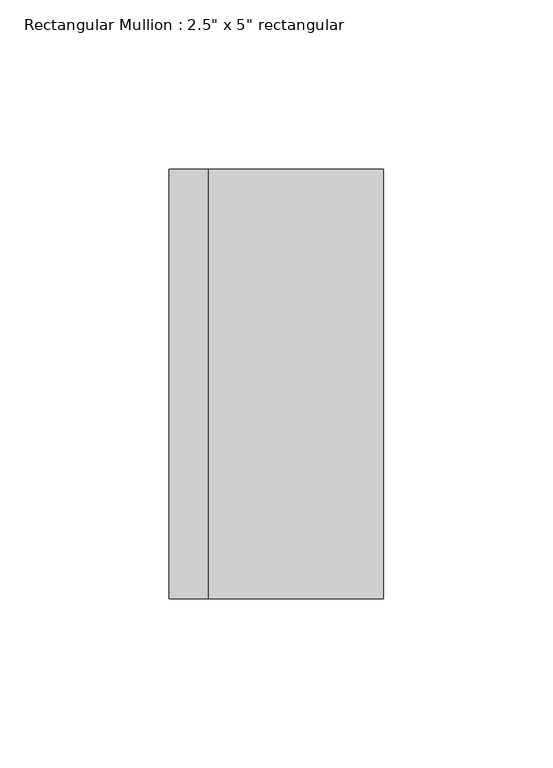
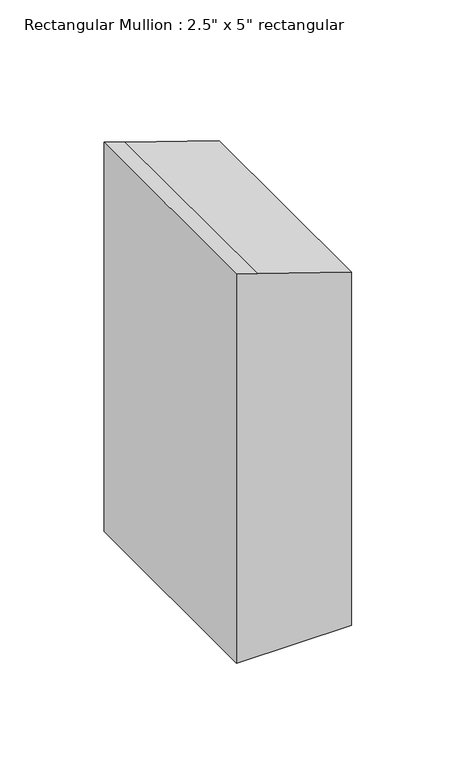
"""IFC4 building model written with IfcOpenShell, lengths in millimetres: member geometry."""

import ifcopenshell
import ifcopenshell.guid

model = None  # the IFC model being written
_history = None  # IfcOwnerHistory: only IFC2X3 demands one
_inside = {}  # id of a spatial element -> (the spatial element, [elements in it])
_under = {}  # id of a project, library or spatial element -> (it, [spatial elements below it])
_declared = {}  # id of a project -> (the project, [libraries it declares])
_typed = {}  # id of a type object -> (the type object, [elements of that type])
_made_of = {}  # id of a material, layer set ... -> (it, [elements and type objects made of it])


def new_model(schema):
    """Start an empty IFC model of exactly this schema.

    Asked for "IFC4X3", IfcOpenShell would pick the latest addendum, in which some entities
    have other attributes; the version numbers below select the first issue.
    IFC2X3 requires an IfcOwnerHistory on every rooted entity: one is made here for all.
    """
    global model, _history
    if schema == "IFC4X3":
        model = ifcopenshell.file(schema_version=(4, 3, 0, 0))
    else:
        model = ifcopenshell.file(schema=schema)
    _inside.clear()
    _under.clear()
    _declared.clear()
    _typed.clear()
    _made_of.clear()
    _history = None
    if model.schema == "IFC2X3":
        org = make("IfcOrganization", Name="unknown")
        user = make(
            "IfcPersonAndOrganization",
            ThePerson=make("IfcPerson", FamilyName="unknown"),
            TheOrganization=org,
        )
        app = make(
            "IfcApplication",
            ApplicationDeveloper=org,
            Version="unknown",
            ApplicationFullName="unknown",
            ApplicationIdentifier="unknown",
        )
        _history = make(
            "IfcOwnerHistory",
            OwningUser=user,
            OwningApplication=app,
            ChangeAction="ADDED",
            CreationDate=0,
        )
    return model


def make(cls, **values):
    """One entity of the class cls with the attributes given. An attribute that is None is left unset."""
    return model.create_entity(
        cls, **{name: value for name, value in values.items() if value is not None}
    )


def rooted(cls, **values):
    """An entity with a GlobalId (a new one), such as an element, a storey or a relation."""
    return make(cls, GlobalId=ifcopenshell.guid.new(), OwnerHistory=_history, **values)


def si_unit(unit_type, name, prefix=None):
    """IfcSIUnit, for example si_unit("LENGTHUNIT", "METRE", prefix="MILLI")."""
    return make("IfcSIUnit", UnitType=unit_type, Prefix=prefix, Name=name)


def assignment(units):
    """IfcUnitAssignment: the units of a project."""
    return None if units is None else make("IfcUnitAssignment", Units=units)


def point(xyz):
    """IfcCartesianPoint."""
    return None if xyz is None else make("IfcCartesianPoint", Coordinates=xyz)


def direction(xyz):
    """IfcDirection."""
    return None if xyz is None else make("IfcDirection", DirectionRatios=xyz)


def frame(location, z_axis=None, x_axis=None):
    """IfcAxis2Placement3D, a coordinate frame: its origin and axes. An axis left out is left unset."""
    return make(
        "IfcAxis2Placement3D",
        Location=point(location),
        Axis=direction(z_axis),
        RefDirection=direction(x_axis),
    )


def origin():
    """The frame at (0, 0, 0) with its axes left unset."""
    return frame((0.0, 0.0, 0.0))


def place(relative_to, where):
    """IfcLocalPlacement: puts the frame where relative to a parent placement (None: the world)."""
    return make(
        "IfcLocalPlacement", PlacementRelTo=relative_to, RelativePlacement=where
    )


def context(
    kind, dimensions, precision=None, world=None, true_north=None, identifier=None
):
    """IfcGeometricRepresentationContext, for example the 3D "Model" context."""
    return make(
        "IfcGeometricRepresentationContext",
        ContextIdentifier=identifier,
        ContextType=kind,
        CoordinateSpaceDimension=dimensions,
        Precision=precision,
        WorldCoordinateSystem=world,
        TrueNorth=true_north,
    )


def project(units=None, contexts=None):
    """IfcProject with its units and contexts."""
    return rooted(
        "IfcProject",
        Name="project",
        RepresentationContexts=contexts,
        UnitsInContext=assignment(units),
    )


def spatial(cls, under=None, at=None, **own):
    """A site, building, storey or space (cls), placed at a placement, below another one or the project."""
    s = rooted(cls, ObjectPlacement=at, **own)
    if under is not None:
        _under.setdefault(under.id(), (under, []))[1].append(s)
    return s


def polyline(points):
    """IfcPolyline through the points."""
    return make("IfcPolyline", Points=[point(p) for p in points])


def outline(outer, holes=None, kind="AREA"):
    """IfcArbitraryClosedProfileDef: a profile drawn as a closed curve; with holes, ...WithVoids."""
    if holes is None:
        return make("IfcArbitraryClosedProfileDef", ProfileType=kind, OuterCurve=outer)
    return make(
        "IfcArbitraryProfileDefWithVoids",
        ProfileType=kind,
        OuterCurve=outer,
        InnerCurves=holes,
    )


def extrude(swept, where, along, depth):
    """IfcExtrudedAreaSolid: the profile swept, set in the frame where, extruded along a direction by depth."""
    return make(
        "IfcExtrudedAreaSolid",
        SweptArea=swept,
        Position=where,
        ExtrudedDirection=direction(along),
        Depth=depth,
    )


def shape(context_of_items, identifier, shape_type, items):
    """IfcShapeRepresentation: the items that make up one representation, for example the "Body"."""
    return make(
        "IfcShapeRepresentation",
        ContextOfItems=context_of_items,
        RepresentationIdentifier=identifier,
        RepresentationType=shape_type,
        Items=items,
    )


def source(mapping_origin, context_of_items, identifier, shape_type, items):
    """IfcRepresentationMap: a shape defined once, which mapped items show again and again."""
    return make(
        "IfcRepresentationMap",
        MappingOrigin=mapping_origin,
        MappedRepresentation=shape(context_of_items, identifier, shape_type, items),
    )


def transform(
    local_origin,
    x_axis=None,
    y_axis=None,
    z_axis=None,
    scale=None,
    scale2=None,
    scale3=None,
    uniform=True,
):
    """IfcCartesianTransformationOperator3D, or its non-uniform kind. x_axis, y_axis, z_axis: its Axis1, 2, 3."""
    if uniform:
        return make(
            "IfcCartesianTransformationOperator3D",
            Axis1=direction(x_axis),
            Axis2=direction(y_axis),
            LocalOrigin=point(local_origin),
            Scale=scale,
            Axis3=direction(z_axis),
        )
    return make(
        "IfcCartesianTransformationOperator3DnonUniform",
        Axis1=direction(x_axis),
        Axis2=direction(y_axis),
        LocalOrigin=point(local_origin),
        Scale=scale,
        Axis3=direction(z_axis),
        Scale2=scale2,
        Scale3=scale3,
    )


def mapped(mapping_source, mapping_target):
    """IfcMappedItem: shows the shape of a source again, moved by a transform."""
    return make(
        "IfcMappedItem", MappingSource=mapping_source, MappingTarget=mapping_target
    )


def made_of(thing, what):
    """Note that an element or type object is made of a material, layer set ...; save() writes the relation."""
    if what is not None:
        _made_of.setdefault(what.id(), (what, []))[1].append(thing)
    return thing


def element(
    cls,
    number,
    at=None,
    inside=None,
    cuts=None,
    type_object=None,
    material=None,
    context=None,
    identifier="Body",
    shape_type=None,
    held_by="IfcProductDefinitionShape",
    body=None,
    shapes=None,
    **own,
):
    """One element of the class cls, such as IfcWall. Its Tag is "e" and its number.

    at: its placement. inside: the storey or other place that contains it. cuts: it is an
    opening in that element (IfcRelVoidsElement). A single representation is given by context,
    identifier, shape_type and body (its items); several are given by shapes. held_by: the class
    of the entity that holds the representations. save() writes the other relations.
    """
    e = rooted(cls, Tag="e%d" % number, ObjectPlacement=at, **own)
    if body is not None:
        shapes = [shape(context, identifier, shape_type, body)]
    if shapes is not None:
        e.Representation = make(held_by, Representations=shapes)
    if inside is not None:
        _inside.setdefault(inside.id(), (inside, []))[1].append(e)
    if cuts is not None:
        rooted(
            "IfcRelVoidsElement", RelatingBuildingElement=cuts, RelatedOpeningElement=e
        )
    if type_object is not None:
        _typed.setdefault(type_object.id(), (type_object, []))[1].append(e)
    return made_of(e, material)


def aggregate(whole, parts):
    """IfcRelAggregates: a whole, such as a stair, and the parts it consists of."""
    return rooted("IfcRelAggregates", RelatingObject=whole, RelatedObjects=parts)


def save(model, path):
    """Write the relations noted so far, then the file.

    IfcRelAggregates (storeys below a building ...), IfcRelContainedInSpatialStructure (elements
    in a storey), IfcRelDefinesByType, IfcRelAssociatesMaterial and IfcRelDeclares: one each for
    every whole, place, type object, material and project.
    """
    for whole, parts in _under.values():
        aggregate(whole, parts)
    for where, things in _inside.values():
        rooted(
            "IfcRelContainedInSpatialStructure",
            RelatedElements=things,
            RelatingStructure=where,
        )
    for kind, things in _typed.values():
        rooted("IfcRelDefinesByType", RelatedObjects=things, RelatingType=kind)
    for what, things in _made_of.values():
        rooted("IfcRelAssociatesMaterial", RelatedObjects=things, RelatingMaterial=what)
    for by, libraries in _declared.values():
        rooted("IfcRelDeclares", RelatingContext=by, RelatedDefinitions=libraries)
    model.write(path)


def member_a66a3142(model_context):
    return source(origin(), model_context, "Body", "SweptSolid", [
        extrude(outline(polyline([(-77.5182105, 31.75), (-60.2413894, -20.0804631), (-56.3515438, -31.75), (-284.0792564, -31.75), (-284.0792564, 31.75), (-77.5182105, 31.75)])), frame((0.0, -63.5, 0.0), z_axis=(0.0, 1.0, 0.0), x_axis=(0.0, 0.0, 1.0)), (0.0, 0.0, 1.0), 127.0),
    ])


if __name__ == "__main__":
    model = new_model("IFC4")
    model_context = context("Model", 3, world=origin())
    ifc_project = project(units=[si_unit("LENGTHUNIT", "METRE", prefix="MILLI")], contexts=[model_context])
    site = spatial("IfcSite", under=ifc_project)
    building = spatial("IfcBuilding", under=site)
    placement = place(None, origin())
    member_shape = member_a66a3142(model_context)
    element("IfcMember", 1, ObjectType="Rectangular Mullion : 2.5\" x 5\" rectangular", at=placement, inside=building, context=model_context, shape_type="MappedRepresentation", body=[
        mapped(member_shape, transform((0.0, 0.0, 0.0), x_axis=(1.0, 0.0, 0.0), y_axis=(0.0, 1.0, 0.0), z_axis=(0.0, 0.0, 1.0))),
    ])
    save(model, "model.ifc")

# Revit data of these elements
# Type "Rectangular Mullion : 2.5\" x 5\" rectangular"
#   built-in parameter 1007304 = 0.416667 (stored number, unit not read)
#   built-in parameter 1007301 = 0.104167 (stored number, unit not read)
#   built-in parameter 1007300 = 0.104167 (stored number, unit not read)
# Element 1 (IfcMember, "Rectangular Mullion : 2.5\" x 5\" rectangular")
#   Materials on its faces: "Metal - Aluminum"
# Materials
#   "Metal - Aluminum": class "Metal", colour RGB 140 140 140, transparency 0
